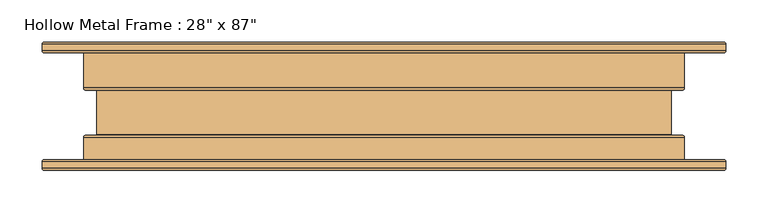
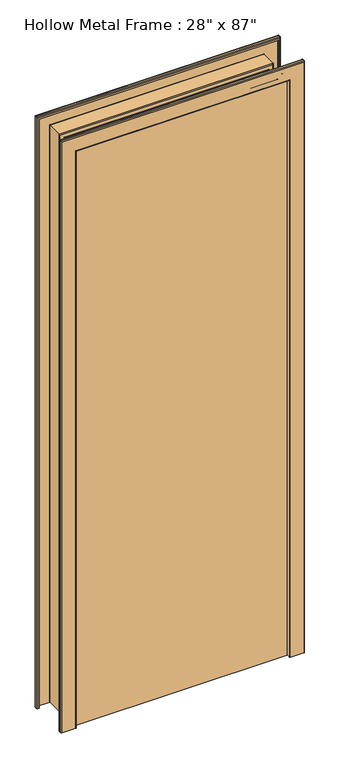
"""IFC4 building model written with IfcOpenShell, lengths in millimetres: door geometry."""

from ifc_helpers import new_model, si_unit, frame, origin, origin_with_axes, place, context, project, spatial, polyline, circle_curve, ellipse_curve, outline, extrude, source, transform, mapped, element, save
from ifc_brep_helpers import plane_surface, cylinder_surface, revolved_surface, advanced_brep


def door_ccd68c71(model_context):
    return source(origin(), model_context, "Body", "SolidModel", [
        advanced_brep(
        [(-403.82825, 63.5635, 0.0), (-406.4, 66.13525, 0.0), (-406.4, 73.66, 0.0), (-403.82825, 76.23175, 0.0), (-358.17175, 76.23175, 0.0), (-355.6, 73.66, 0.0), (-355.6, 21.68525, 0.0), (-354.584, 20.66925, 0.0), (-342.29675, 20.66925, 0.0), (-339.725, 18.0975, 0.0), (-339.725, -33.6931, 0.0), (-342.29675, -36.26485, 0.0), (-354.584, -36.26485, 0.0), (-355.6, -37.28085, 0.0), (-355.6, -73.5965, 0.0), (-358.17175, -76.16825, 0.0), (-403.82825, -76.16825, 0.0), (-406.4, -73.5965, 0.0), (-406.4, -66.07175, 0.0), (-403.82825, -63.5, 0.0), (-398.4625, -63.5, 0.0), (-398.4625, -65.05575, 0.0), (-403.82825, -65.05575, 0.0), (-404.84425, -66.07175, 0.0), (-404.84425, -73.5965, 0.0), (-403.82825, -74.6125, 0.0), (-358.17175, -74.6125, 0.0), (-357.15575, -73.5965, 0.0), (-357.15575, -37.28085, 0.0), (-354.584, -34.7091, 0.0), (-342.29675, -34.7091, 0.0), (-341.28075, -33.6931, 0.0), (-341.28075, 18.0975, 0.0), (-342.29675, 19.1135, 0.0), (-354.584, 19.1135, 0.0), (-357.15575, 21.68525, 0.0), (-357.15575, 73.66, 0.0), (-358.17175, 74.676, 0.0), (-403.82825, 74.676, 0.0), (-404.84425, 73.66, 0.0), (-404.84425, 66.13525, 0.0), (-403.82825, 65.11925, 0.0), (-398.4625, 65.11925, 0.0), (-398.4625, 63.5635, 0.0), (-403.82825, 63.5635, 2080.2282501), (-406.4, 66.13525, 2082.8000001), (-406.4, 73.66, 2082.8000001), (-403.82825, 76.23175, 2080.2282501), (403.82825, 76.23175, 2080.2282501), (403.82825, 76.23175, 0.0), (358.17175, 76.23175, 0.0), (358.17175, 76.23175, 2034.5717501), (-358.17175, 76.23175, 2034.5717501), (-355.6, 73.66, 2032.0000001), (-355.6, 21.68525, 2032.0000001), (-354.584, 20.66925, 2030.9840001), (354.584, 20.66925, 2030.9840001), (354.584, 20.66925, 0.0), (342.29675, 20.66925, 0.0), (342.29675, 20.66925, 2018.6967501), (-342.29675, 20.66925, 2018.6967501), (-339.725, 18.0975, 2016.1250001), (-339.725, -33.6931, 2016.1250001), (-342.29675, -36.26485, 2018.6967501), (342.29675, -36.26485, 2018.6967501), (342.29675, -36.26485, 0.0), (354.584, -36.26485, 0.0), (354.584, -36.26485, 2030.9840001), (-354.584, -36.26485, 2030.9840001), (-355.6, -37.28085, 2032.0000001), (-355.6, -73.5965, 2032.0000001), (-358.17175, -76.16825, 2034.5717501), (358.17175, -76.16825, 2034.5717501), (358.17175, -76.16825, 0.0), (403.82825, -76.16825, 0.0), (403.82825, -76.16825, 2080.2282501), (-403.82825, -76.16825, 2080.2282501), (-406.4, -73.5965, 2082.8000001), (-406.4, -66.07175, 2082.8000001), (-403.82825, -63.5, 2080.2282501), (403.82825, -63.5, 2080.2282501), (403.82825, -63.5, 0.0), (398.4625, -63.5, 0.0), (398.4625, -63.5, 2074.8625001), (-398.4625, -63.5, 2074.8625001), (-398.4625, -65.05575, 2074.8625001), (398.4625, -65.05575, 2074.8625001), (398.4625, -65.05575, 0.0), (403.82825, -65.05575, 0.0), (403.82825, -65.05575, 2080.2282501), (-403.82825, -65.05575, 2080.2282501), (-404.84425, -66.07175, 2081.2442501), (-404.84425, -73.5965, 2081.2442501), (-403.82825, -74.6125, 2080.2282501), (403.82825, -74.6125, 2080.2282501), (403.82825, -74.6125, 0.0), (358.17175, -74.6125, 0.0), (358.17175, -74.6125, 2034.5717501), (-358.17175, -74.6125, 2034.5717501), (-357.15575, -73.5965, 2033.5557501), (-357.15575, -37.28085, 2033.5557501), (-354.584, -34.7091, 2030.9840001), (354.584, -34.7091, 2030.9840001), (354.584, -34.7091, 0.0), (342.29675, -34.7091, 0.0), (342.29675, -34.7091, 2018.6967501), (-342.29675, -34.7091, 2018.6967501), (-341.28075, -33.6931, 2017.6807501), (-341.28075, 18.0975, 2017.6807501), (-342.29675, 19.1135, 2018.6967501), (342.29675, 19.1135, 2018.6967501), (342.29675, 19.1135, 0.0), (354.584, 19.1135, 0.0), (354.584, 19.1135, 2030.9840001), (-354.584, 19.1135, 2030.9840001), (-357.15575, 21.68525, 2033.5557501), (-357.15575, 73.66, 2033.5557501), (-358.17175, 74.676, 2034.5717501), (358.17175, 74.676, 2034.5717501), (358.17175, 74.676, 0.0), (403.82825, 74.676, 0.0), (403.82825, 74.676, 2080.2282501), (-403.82825, 74.676, 2080.2282501), (-404.84425, 73.66, 2081.2442501), (-404.84425, 66.13525, 2081.2442501), (-403.82825, 65.11925, 2080.2282501), (403.82825, 65.11925, 2080.2282501), (403.82825, 65.11925, 0.0), (398.4625, 65.11925, 0.0), (398.4625, 65.11925, 2074.8625001), (-398.4625, 65.11925, 2074.8625001), (-398.4625, 63.5635, 2074.8625001), (398.4625, 63.5635, 2074.8625001), (398.4625, 63.5635, 0.0), (403.82825, 63.5635, 0.0), (403.82825, 63.5635, 2080.2282501), (406.4, 66.13525, 2082.8000001), (406.4, 73.66, 2082.8000001), (355.6, 73.66, 2032.0000001), (355.6, 21.68525, 2032.0000001), (339.725, 18.0975, 2016.1250001), (339.725, -33.6931, 2016.1250001), (355.6, -37.28085, 2032.0000001), (355.6, -73.5965, 2032.0000001), (406.4, -73.5965, 2082.8000001), (406.4, -66.07175, 2082.8000001), (404.84425, -66.07175, 2081.2442501), (404.84425, -73.5965, 2081.2442501), (357.15575, -73.5965, 2033.5557501), (357.15575, -37.28085, 2033.5557501), (341.28075, -33.6931, 2017.6807501), (341.28075, 18.0975, 2017.6807501), (357.15575, 21.68525, 2033.5557501), (357.15575, 73.66, 2033.5557501), (404.84425, 73.66, 2081.2442501), (404.84425, 66.13525, 2081.2442501), (404.84425, 66.13525, 0.0), (404.84425, 73.66, 0.0), (357.15575, 73.66, 0.0), (357.15575, 21.68525, 0.0), (341.28075, 18.0975, 0.0), (341.28075, -33.6931, 0.0), (357.15575, -37.28085, 0.0), (357.15575, -73.5965, 0.0), (404.84425, -73.5965, 0.0), (404.84425, -66.07175, 0.0), (406.4, -66.07175, 0.0), (406.4, -73.5965, 0.0), (355.6, -73.5965, 0.0), (355.6, -37.28085, 0.0), (339.725, -33.6931, 0.0), (339.725, 18.0975, 0.0), (355.6, 21.68525, 0.0), (355.6, 73.66, 0.0), (406.4, 73.66, 0.0), (406.4, 66.13525, 0.0)],
        [
            (0, 1, circle_curve(frame((-403.82825, 66.13525, 0.0), z_axis=(0.0, 0.0, -1.0), x_axis=(0.0, -1.0, 0.0)), 2.57175)),
            (1, 2),
            (2, 3, circle_curve(frame((-403.82825, 73.66, 0.0), z_axis=(0.0, 0.0, -1.0), x_axis=(0.0, -1.0, 0.0)), 2.57175)),
            (3, 4),
            (4, 5, circle_curve(frame((-358.17175, 73.66, 0.0), z_axis=(0.0, 0.0, -1.0), x_axis=(0.0, -1.0, 0.0)), 2.57175)),
            (5, 6),
            (6, 7, circle_curve(frame((-354.584, 21.68525, 0.0), z_axis=(0.0, 0.0, 1.0), x_axis=(0.0, -1.0, 0.0)), 1.016)),
            (7, 8),
            (8, 9, circle_curve(frame((-342.29675, 18.0975, 0.0), z_axis=(0.0, 0.0, -1.0), x_axis=(0.0, -1.0, 0.0)), 2.57175)),
            (9, 10),
            (10, 11, circle_curve(frame((-342.29675, -33.6931, 0.0), z_axis=(0.0, 0.0, -1.0), x_axis=(0.0, -1.0, 0.0)), 2.57175)),
            (11, 12),
            (12, 13, circle_curve(frame((-354.584, -37.28085, 0.0), z_axis=(0.0, 0.0, 1.0), x_axis=(0.0, -1.0, 0.0)), 1.016)),
            (13, 14),
            (14, 15, circle_curve(frame((-358.17175, -73.5965, 0.0), z_axis=(0.0, 0.0, -1.0), x_axis=(0.0, -1.0, 0.0)), 2.57175)),
            (15, 16),
            (16, 17, circle_curve(frame((-403.82825, -73.5965, 0.0), z_axis=(0.0, 0.0, -1.0), x_axis=(0.0, -1.0, 0.0)), 2.57175)),
            (17, 18),
            (18, 19, circle_curve(frame((-403.82825, -66.07175, 0.0), z_axis=(0.0, 0.0, -1.0), x_axis=(0.0, -1.0, 0.0)), 2.57175)),
            (19, 20),
            (20, 21),
            (21, 22),
            (22, 23, circle_curve(frame((-403.82825, -66.07175, 0.0), z_axis=(0.0, 0.0, 1.0), x_axis=(0.0, -1.0, 0.0)), 1.016)),
            (23, 24),
            (24, 25, circle_curve(frame((-403.82825, -73.5965, 0.0), z_axis=(0.0, 0.0, 1.0), x_axis=(0.0, -1.0, 0.0)), 1.016)),
            (25, 26),
            (26, 27, circle_curve(frame((-358.17175, -73.5965, 0.0), z_axis=(0.0, 0.0, 1.0), x_axis=(0.0, -1.0, 0.0)), 1.016)),
            (27, 28),
            (28, 29, circle_curve(frame((-354.584, -37.28085, 0.0), z_axis=(0.0, 0.0, -1.0), x_axis=(0.0, -1.0, 0.0)), 2.57175)),
            (29, 30),
            (30, 31, circle_curve(frame((-342.29675, -33.6931, 0.0), z_axis=(0.0, 0.0, 1.0), x_axis=(0.0, -1.0, 0.0)), 1.016)),
            (31, 32),
            (32, 33, circle_curve(frame((-342.29675, 18.0975, 0.0), z_axis=(0.0, 0.0, 1.0), x_axis=(0.0, -1.0, 0.0)), 1.016)),
            (33, 34),
            (34, 35, circle_curve(frame((-354.584, 21.68525, 0.0), z_axis=(0.0, 0.0, -1.0), x_axis=(0.0, -1.0, 0.0)), 2.57175)),
            (35, 36),
            (36, 37, circle_curve(frame((-358.17175, 73.66, 0.0), z_axis=(0.0, 0.0, 1.0), x_axis=(0.0, -1.0, 0.0)), 1.016)),
            (37, 38),
            (38, 39, circle_curve(frame((-403.82825, 73.66, 0.0), z_axis=(0.0, 0.0, 1.0), x_axis=(0.0, -1.0, 0.0)), 1.016)),
            (39, 40),
            (40, 41, circle_curve(frame((-403.82825, 66.13525, 0.0), z_axis=(0.0, 0.0, 1.0), x_axis=(0.0, -1.0, 0.0)), 1.016)),
            (41, 42),
            (42, 43),
            (43, 0),
            (0, 44),
            (44, 45, ellipse_curve(frame((-403.82825, 66.13525, 2080.2282501), z_axis=(-0.7071067811865475, 0.0, -0.7071067811865475), x_axis=(0.7071067811865474, 0.0, -0.7071067811865476)), 3.6370037, 2.57175)),
            (45, 1),
            (45, 46),
            (46, 2),
            (46, 47, ellipse_curve(frame((-403.82825, 73.66, 2080.2282501), z_axis=(-0.7071067811865475, 0.0, -0.7071067811865475), x_axis=(0.7071067811865474, 0.0, -0.7071067811865476)), 3.6370037, 2.57175)),
            (47, 3),
            (47, 48),
            (48, 49),
            (49, 50),
            (50, 51),
            (51, 52),
            (52, 4),
            (52, 53, ellipse_curve(frame((-358.17175, 73.66, 2034.5717501), z_axis=(-0.7071067811865475, 0.0, -0.7071067811865475), x_axis=(0.7071067811865474, 0.0, -0.7071067811865476)), 3.6370037, 2.57175)),
            (53, 5),
            (53, 54),
            (54, 6),
            (54, 55, ellipse_curve(frame((-354.584, 21.68525, 2030.9840001), z_axis=(0.7071067811865475, 0.0, 0.7071067811865475), x_axis=(-0.7071067811865474, 0.0, 0.7071067811865476)), 1.436841, 1.016)),
            (55, 7),
            (55, 56),
            (56, 57),
            (57, 58),
            (58, 59),
            (59, 60),
            (60, 8),
            (60, 61, ellipse_curve(frame((-342.29675, 18.0975, 2018.6967501), z_axis=(-0.7071067811865475, 0.0, -0.7071067811865475), x_axis=(0.7071067811865474, 0.0, -0.7071067811865476)), 3.6370037, 2.57175)),
            (61, 9),
            (61, 62),
            (62, 10),
            (62, 63, ellipse_curve(frame((-342.29675, -33.6931, 2018.6967501), z_axis=(-0.7071067811865475, 0.0, -0.7071067811865475), x_axis=(0.7071067811865474, 0.0, -0.7071067811865476)), 3.6370037, 2.57175)),
            (63, 11),
            (63, 64),
            (64, 65),
            (65, 66),
            (66, 67),
            (67, 68),
            (68, 12),
            (68, 69, ellipse_curve(frame((-354.584, -37.28085, 2030.9840001), z_axis=(0.7071067811865475, 0.0, 0.7071067811865475), x_axis=(-0.7071067811865474, 0.0, 0.7071067811865476)), 1.436841, 1.016)),
            (69, 13),
            (69, 70),
            (70, 14),
            (70, 71, ellipse_curve(frame((-358.17175, -73.5965, 2034.5717501), z_axis=(-0.7071067811865475, 0.0, -0.7071067811865475), x_axis=(0.7071067811865474, 0.0, -0.7071067811865476)), 3.6370037, 2.57175)),
            (71, 15),
            (71, 72),
            (72, 73),
            (73, 74),
            (74, 75),
            (75, 76),
            (76, 16),
            (76, 77, ellipse_curve(frame((-403.82825, -73.5965, 2080.2282501), z_axis=(-0.7071067811865475, 0.0, -0.7071067811865475), x_axis=(0.7071067811865474, 0.0, -0.7071067811865476)), 3.6370037, 2.57175)),
            (77, 17),
            (77, 78),
            (78, 18),
            (78, 79, ellipse_curve(frame((-403.82825, -66.07175, 2080.2282501), z_axis=(-0.7071067811865475, 0.0, -0.7071067811865475), x_axis=(0.7071067811865474, 0.0, -0.7071067811865476)), 3.6370037, 2.57175)),
            (79, 19),
            (79, 80),
            (80, 81),
            (81, 82),
            (82, 83),
            (83, 84),
            (84, 20),
            (84, 85),
            (85, 21),
            (85, 86),
            (86, 87),
            (87, 88),
            (88, 89),
            (89, 90),
            (90, 22),
            (90, 91, ellipse_curve(frame((-403.82825, -66.07175, 2080.2282501), z_axis=(0.7071067811865475, 0.0, 0.7071067811865475), x_axis=(-0.7071067811865474, 0.0, 0.7071067811865476)), 1.436841, 1.016)),
            (91, 23),
            (91, 92),
            (92, 24),
            (92, 93, ellipse_curve(frame((-403.82825, -73.5965, 2080.2282501), z_axis=(0.7071067811865475, 0.0, 0.7071067811865475), x_axis=(-0.7071067811865474, 0.0, 0.7071067811865476)), 1.436841, 1.016)),
            (93, 25),
            (93, 94),
            (94, 95),
            (95, 96),
            (96, 97),
            (97, 98),
            (98, 26),
            (98, 99, ellipse_curve(frame((-358.17175, -73.5965, 2034.5717501), z_axis=(0.7071067811865475, 0.0, 0.7071067811865475), x_axis=(-0.7071067811865474, 0.0, 0.7071067811865476)), 1.436841, 1.016)),
            (99, 27),
            (99, 100),
            (100, 28),
            (100, 101, ellipse_curve(frame((-354.584, -37.28085, 2030.9840001), z_axis=(-0.7071067811865475, 0.0, -0.7071067811865475), x_axis=(0.7071067811865474, 0.0, -0.7071067811865476)), 3.6370037, 2.57175)),
            (101, 29),
            (101, 102),
            (102, 103),
            (103, 104),
            (104, 105),
            (105, 106),
            (106, 30),
            (106, 107, ellipse_curve(frame((-342.29675, -33.6931, 2018.6967501), z_axis=(0.7071067811865475, 0.0, 0.7071067811865475), x_axis=(-0.7071067811865474, 0.0, 0.7071067811865476)), 1.436841, 1.016)),
            (107, 31),
            (107, 108),
            (108, 32),
            (108, 109, ellipse_curve(frame((-342.29675, 18.0975, 2018.6967501), z_axis=(0.7071067811865475, 0.0, 0.7071067811865475), x_axis=(-0.7071067811865474, 0.0, 0.7071067811865476)), 1.436841, 1.016)),
            (109, 33),
            (109, 110),
            (110, 111),
            (111, 112),
            (112, 113),
            (113, 114),
            (114, 34),
            (114, 115, ellipse_curve(frame((-354.584, 21.68525, 2030.9840001), z_axis=(-0.7071067811865475, 0.0, -0.7071067811865475), x_axis=(0.7071067811865474, 0.0, -0.7071067811865476)), 3.6370037, 2.57175)),
            (115, 35),
            (115, 116),
            (116, 36),
            (116, 117, ellipse_curve(frame((-358.17175, 73.66, 2034.5717501), z_axis=(0.7071067811865475, 0.0, 0.7071067811865475), x_axis=(-0.7071067811865474, 0.0, 0.7071067811865476)), 1.436841, 1.016)),
            (117, 37),
            (117, 118),
            (118, 119),
            (119, 120),
            (120, 121),
            (121, 122),
            (122, 38),
            (122, 123, ellipse_curve(frame((-403.82825, 73.66, 2080.2282501), z_axis=(0.7071067811865475, 0.0, 0.7071067811865475), x_axis=(-0.7071067811865474, 0.0, 0.7071067811865476)), 1.436841, 1.016)),
            (123, 39),
            (123, 124),
            (124, 40),
            (124, 125, ellipse_curve(frame((-403.82825, 66.13525, 2080.2282501), z_axis=(0.7071067811865475, 0.0, 0.7071067811865475), x_axis=(-0.7071067811865474, 0.0, 0.7071067811865476)), 1.436841, 1.016)),
            (125, 41),
            (125, 126),
            (126, 127),
            (127, 128),
            (128, 129),
            (129, 130),
            (130, 42),
            (130, 131),
            (131, 43),
            (131, 132),
            (132, 133),
            (133, 134),
            (134, 135),
            (135, 44),
            (135, 136, ellipse_curve(frame((403.82825, 66.13525, 2080.2282501), z_axis=(-0.7071067811865475, 0.0, 0.7071067811865475), x_axis=(-0.7071067811865476, 0.0, -0.7071067811865474)), 3.6370037, 2.57175)),
            (136, 45),
            (136, 137),
            (137, 46),
            (137, 48, ellipse_curve(frame((403.82825, 73.66, 2080.2282501), z_axis=(-0.7071067811865475, 0.0, 0.7071067811865475), x_axis=(-0.7071067811865476, 0.0, -0.7071067811865474)), 3.6370037, 2.57175)),
            (51, 138, ellipse_curve(frame((358.17175, 73.66, 2034.5717501), z_axis=(-0.7071067811865475, 0.0, 0.7071067811865475), x_axis=(-0.7071067811865476, 0.0, -0.7071067811865474)), 3.6370037, 2.57175)),
            (138, 53),
            (138, 139),
            (139, 54),
            (139, 56, ellipse_curve(frame((354.584, 21.68525, 2030.9840001), z_axis=(0.7071067811865475, 0.0, -0.7071067811865475), x_axis=(0.7071067811865476, 0.0, 0.7071067811865474)), 1.436841, 1.016)),
            (59, 140, ellipse_curve(frame((342.29675, 18.0975, 2018.6967501), z_axis=(-0.7071067811865475, 0.0, 0.7071067811865475), x_axis=(-0.7071067811865476, 0.0, -0.7071067811865474)), 3.6370037, 2.57175)),
            (140, 61),
            (140, 141),
            (141, 62),
            (141, 64, ellipse_curve(frame((342.29675, -33.6931, 2018.6967501), z_axis=(-0.7071067811865475, 0.0, 0.7071067811865475), x_axis=(-0.7071067811865476, 0.0, -0.7071067811865474)), 3.6370037, 2.57175)),
            (67, 142, ellipse_curve(frame((354.584, -37.28085, 2030.9840001), z_axis=(0.7071067811865475, 0.0, -0.7071067811865475), x_axis=(0.7071067811865476, 0.0, 0.7071067811865474)), 1.436841, 1.016)),
            (142, 69),
            (142, 143),
            (143, 70),
            (143, 72, ellipse_curve(frame((358.17175, -73.5965, 2034.5717501), z_axis=(-0.7071067811865475, 0.0, 0.7071067811865475), x_axis=(-0.7071067811865476, 0.0, -0.7071067811865474)), 3.6370037, 2.57175)),
            (75, 144, ellipse_curve(frame((403.82825, -73.5965, 2080.2282501), z_axis=(-0.7071067811865475, 0.0, 0.7071067811865475), x_axis=(-0.7071067811865476, 0.0, -0.7071067811865474)), 3.6370037, 2.57175)),
            (144, 77),
            (144, 145),
            (145, 78),
            (145, 80, ellipse_curve(frame((403.82825, -66.07175, 2080.2282501), z_axis=(-0.7071067811865475, 0.0, 0.7071067811865475), x_axis=(-0.7071067811865476, 0.0, -0.7071067811865474)), 3.6370037, 2.57175)),
            (83, 86),
            (89, 146, ellipse_curve(frame((403.82825, -66.07175, 2080.2282501), z_axis=(0.7071067811865475, 0.0, -0.7071067811865475), x_axis=(0.7071067811865476, 0.0, 0.7071067811865474)), 1.436841, 1.016)),
            (146, 91),
            (146, 147),
            (147, 92),
            (147, 94, ellipse_curve(frame((403.82825, -73.5965, 2080.2282501), z_axis=(0.7071067811865475, 0.0, -0.7071067811865475), x_axis=(0.7071067811865476, 0.0, 0.7071067811865474)), 1.436841, 1.016)),
            (97, 148, ellipse_curve(frame((358.17175, -73.5965, 2034.5717501), z_axis=(0.7071067811865475, 0.0, -0.7071067811865475), x_axis=(0.7071067811865476, 0.0, 0.7071067811865474)), 1.436841, 1.016)),
            (148, 99),
            (148, 149),
            (149, 100),
            (149, 102, ellipse_curve(frame((354.584, -37.28085, 2030.9840001), z_axis=(-0.7071067811865475, 0.0, 0.7071067811865475), x_axis=(-0.7071067811865476, 0.0, -0.7071067811865474)), 3.6370037, 2.57175)),
            (105, 150, ellipse_curve(frame((342.29675, -33.6931, 2018.6967501), z_axis=(0.7071067811865475, 0.0, -0.7071067811865475), x_axis=(0.7071067811865476, 0.0, 0.7071067811865474)), 1.436841, 1.016)),
            (150, 107),
            (150, 151),
            (151, 108),
            (151, 110, ellipse_curve(frame((342.29675, 18.0975, 2018.6967501), z_axis=(0.7071067811865475, 0.0, -0.7071067811865475), x_axis=(0.7071067811865476, 0.0, 0.7071067811865474)), 1.436841, 1.016)),
            (113, 152, ellipse_curve(frame((354.584, 21.68525, 2030.9840001), z_axis=(-0.7071067811865475, 0.0, 0.7071067811865475), x_axis=(-0.7071067811865476, 0.0, -0.7071067811865474)), 3.6370037, 2.57175)),
            (152, 115),
            (152, 153),
            (153, 116),
            (153, 118, ellipse_curve(frame((358.17175, 73.66, 2034.5717501), z_axis=(0.7071067811865475, 0.0, -0.7071067811865475), x_axis=(0.7071067811865476, 0.0, 0.7071067811865474)), 1.436841, 1.016)),
            (121, 154, ellipse_curve(frame((403.82825, 73.66, 2080.2282501), z_axis=(0.7071067811865475, 0.0, -0.7071067811865475), x_axis=(0.7071067811865476, 0.0, 0.7071067811865474)), 1.436841, 1.016)),
            (154, 123),
            (154, 155),
            (155, 124),
            (155, 126, ellipse_curve(frame((403.82825, 66.13525, 2080.2282501), z_axis=(0.7071067811865475, 0.0, -0.7071067811865475), x_axis=(0.7071067811865476, 0.0, 0.7071067811865474)), 1.436841, 1.016)),
            (129, 132),
            (133, 128),
            (127, 156, circle_curve(frame((403.82825, 66.13525, 0.0), z_axis=(0.0, 0.0, 1.0), x_axis=(0.0, -1.0, 0.0)), 1.016)),
            (156, 157),
            (157, 120, circle_curve(frame((403.82825, 73.66, 0.0), z_axis=(0.0, 0.0, 1.0), x_axis=(0.0, -1.0, 0.0)), 1.016)),
            (119, 158, circle_curve(frame((358.17175, 73.66, 0.0), z_axis=(0.0, 0.0, 1.0), x_axis=(0.0, -1.0, 0.0)), 1.016)),
            (158, 159),
            (159, 112, circle_curve(frame((354.584, 21.68525, 0.0), z_axis=(0.0, 0.0, -1.0), x_axis=(0.0, -1.0, 0.0)), 2.57175)),
            (111, 160, circle_curve(frame((342.29675, 18.0975, 0.0), z_axis=(0.0, 0.0, 1.0), x_axis=(0.0, -1.0, 0.0)), 1.016)),
            (160, 161),
            (161, 104, circle_curve(frame((342.29675, -33.6931, 0.0), z_axis=(0.0, 0.0, 1.0), x_axis=(0.0, -1.0, 0.0)), 1.016)),
            (103, 162, circle_curve(frame((354.584, -37.28085, 0.0), z_axis=(0.0, 0.0, -1.0), x_axis=(0.0, -1.0, 0.0)), 2.57175)),
            (162, 163),
            (163, 96, circle_curve(frame((358.17175, -73.5965, 0.0), z_axis=(0.0, 0.0, 1.0), x_axis=(0.0, -1.0, 0.0)), 1.016)),
            (95, 164, circle_curve(frame((403.82825, -73.5965, 0.0), z_axis=(0.0, 0.0, 1.0), x_axis=(0.0, -1.0, 0.0)), 1.016)),
            (164, 165),
            (165, 88, circle_curve(frame((403.82825, -66.07175, 0.0), z_axis=(0.0, 0.0, 1.0), x_axis=(0.0, -1.0, 0.0)), 1.016)),
            (87, 82),
            (81, 166, circle_curve(frame((403.82825, -66.07175, 0.0), z_axis=(0.0, 0.0, -1.0), x_axis=(0.0, -1.0, 0.0)), 2.57175)),
            (166, 167),
            (167, 74, circle_curve(frame((403.82825, -73.5965, 0.0), z_axis=(0.0, 0.0, -1.0), x_axis=(0.0, -1.0, 0.0)), 2.57175)),
            (73, 168, circle_curve(frame((358.17175, -73.5965, 0.0), z_axis=(0.0, 0.0, -1.0), x_axis=(0.0, -1.0, 0.0)), 2.57175)),
            (168, 169),
            (169, 66, circle_curve(frame((354.584, -37.28085, 0.0), z_axis=(0.0, 0.0, 1.0), x_axis=(0.0, -1.0, 0.0)), 1.016)),
            (65, 170, circle_curve(frame((342.29675, -33.6931, 0.0), z_axis=(0.0, 0.0, -1.0), x_axis=(0.0, -1.0, 0.0)), 2.57175)),
            (170, 171),
            (171, 58, circle_curve(frame((342.29675, 18.0975, 0.0), z_axis=(0.0, 0.0, -1.0), x_axis=(0.0, -1.0, 0.0)), 2.57175)),
            (57, 172, circle_curve(frame((354.584, 21.68525, 0.0), z_axis=(0.0, 0.0, 1.0), x_axis=(0.0, -1.0, 0.0)), 1.016)),
            (172, 173),
            (173, 50, circle_curve(frame((358.17175, 73.66, 0.0), z_axis=(0.0, 0.0, -1.0), x_axis=(0.0, -1.0, 0.0)), 2.57175)),
            (49, 174, circle_curve(frame((403.82825, 73.66, 0.0), z_axis=(0.0, 0.0, -1.0), x_axis=(0.0, -1.0, 0.0)), 2.57175)),
            (174, 175),
            (175, 134, circle_curve(frame((403.82825, 66.13525, 0.0), z_axis=(0.0, 0.0, -1.0), x_axis=(0.0, -1.0, 0.0)), 2.57175)),
            (175, 136),
            (174, 137),
            (173, 138),
            (172, 139),
            (171, 140),
            (170, 141),
            (169, 142),
            (168, 143),
            (167, 144),
            (166, 145),
            (165, 146),
            (164, 147),
            (163, 148),
            (162, 149),
            (161, 150),
            (160, 151),
            (159, 152),
            (158, 153),
            (157, 154),
            (156, 155),
        ],
        [
            plane_surface(frame((-366.7125, -63.5, 0.0), z_axis=(0.0, 0.0, -1.0), x_axis=(1.0, 0.0, 0.0))),
            cylinder_surface(frame((-403.82825, 66.13525, 0.0), z_axis=(0.0, 0.0, -1.0), x_axis=(0.0, -1.0, 0.0)), 2.57175),
            plane_surface(frame((-406.4, 66.13525, 0.0), z_axis=(-1.0, 0.0, 0.0), x_axis=(0.0, 0.0, 1.0))),
            cylinder_surface(frame((-403.82825, 73.66, 0.0), z_axis=(0.0, 0.0, -1.0), x_axis=(0.0, -1.0, 0.0)), 2.57175),
            plane_surface(frame((-403.82825, 76.23175, 0.0), z_axis=(0.0, 1.0, 0.0), x_axis=(0.0, 0.0, 1.0))),
            cylinder_surface(frame((-358.17175, 73.66, 0.0), z_axis=(0.0, 0.0, -1.0), x_axis=(0.0, -1.0, 0.0)), 2.57175),
            plane_surface(frame((-355.6, 73.66, 0.0), z_axis=(1.0, 0.0, 0.0), x_axis=(0.0, 0.0, 1.0))),
            revolved_surface(polyline([(-354.584, 20.669249999999998, 2032.0000001145868), (-354.584, 20.669249999999998, 0.0)]), (-354.584, 21.68525, 0.0), (0.0, 0.0, 1.0)),
            plane_surface(frame((-354.584, 20.66925, 0.0), z_axis=(0.0, 1.0, 0.0), x_axis=(0.0, 0.0, 1.0))),
            cylinder_surface(frame((-342.29675, 18.0975, 0.0), z_axis=(0.0, 0.0, -1.0), x_axis=(0.0, -1.0, 0.0)), 2.57175),
            plane_surface(frame((-339.725, 18.0975, 0.0), z_axis=(1.0, 0.0, 0.0), x_axis=(0.0, 0.0, 1.0))),
            cylinder_surface(frame((-342.29675, -33.6931, 0.0), z_axis=(0.0, 0.0, -1.0), x_axis=(0.0, -1.0, 0.0)), 2.57175),
            plane_surface(frame((-342.29675, -36.26485, 0.0), z_axis=(0.0, -1.0, 0.0), x_axis=(0.0, 0.0, 1.0))),
            revolved_surface(polyline([(-354.584, -38.29685, 2032.0000001145868), (-354.584, -38.29685, 0.0)]), (-354.584, -37.28085, 0.0), (0.0, 0.0, 1.0)),
            plane_surface(frame((-355.6, -37.28085, 0.0), z_axis=(1.0, 0.0, 0.0), x_axis=(0.0, 0.0, 1.0))),
            cylinder_surface(frame((-358.17175, -73.5965, 0.0), z_axis=(0.0, 0.0, -1.0), x_axis=(0.0, -1.0, 0.0)), 2.57175),
            plane_surface(frame((-358.17175, -76.16825, 0.0), z_axis=(0.0, -1.0, 0.0), x_axis=(0.0, 0.0, 1.0))),
            cylinder_surface(frame((-403.82825, -73.5965, 0.0), z_axis=(0.0, 0.0, -1.0), x_axis=(0.0, -1.0, 0.0)), 2.57175),
            plane_surface(frame((-406.4, -73.5965, 0.0), z_axis=(-1.0, 0.0, 0.0), x_axis=(0.0, 0.0, 1.0))),
            cylinder_surface(frame((-403.82825, -66.07175, 0.0), z_axis=(0.0, 0.0, -1.0), x_axis=(0.0, -1.0, 0.0)), 2.57175),
            plane_surface(frame((-403.82825, -63.5, 0.0), z_axis=(0.0, 1.0, 0.0), x_axis=(0.0, 0.0, 1.0))),
            plane_surface(frame((-398.4625, -63.5, 0.0), z_axis=(1.0, 0.0, 0.0), x_axis=(0.0, 0.0, 1.0))),
            plane_surface(frame((-398.4625, -65.05575, 0.0), z_axis=(0.0, -1.0, 0.0), x_axis=(0.0, 0.0, 1.0))),
            revolved_surface(polyline([(-403.82825, -67.08775, 2081.244250114587), (-403.82825, -67.08775, 0.0)]), (-403.82825, -66.07175, 0.0), (0.0, 0.0, 1.0)),
            plane_surface(frame((-404.84425, -66.07175, 0.0), z_axis=(1.0, 0.0, 0.0), x_axis=(0.0, 0.0, 1.0))),
            revolved_surface(polyline([(-403.82825, -74.61250000000001, 2081.244250114587), (-403.82825, -74.61250000000001, 0.0)]), (-403.82825, -73.5965, 0.0), (0.0, 0.0, 1.0)),
            plane_surface(frame((-403.82825, -74.6125, 0.0), z_axis=(0.0, 1.0, 0.0), x_axis=(0.0, 0.0, 1.0))),
            revolved_surface(polyline([(-358.17175, -74.61250000000001, 2035.5877501145867), (-358.17175, -74.61250000000001, 0.0)]), (-358.17175, -73.5965, 0.0), (0.0, 0.0, 1.0)),
            plane_surface(frame((-357.15575, -73.5965, 0.0), z_axis=(-1.0, 0.0, 0.0), x_axis=(0.0, 0.0, 1.0))),
            cylinder_surface(frame((-354.584, -37.28085, 0.0), z_axis=(0.0, 0.0, -1.0), x_axis=(0.0, -1.0, 0.0)), 2.57175),
            plane_surface(frame((-354.584, -34.7091, 0.0), z_axis=(0.0, 1.0, 0.0), x_axis=(0.0, 0.0, 1.0))),
            revolved_surface(polyline([(-342.29675, -34.7091, 2019.7127501145867), (-342.29675, -34.7091, 0.0)]), (-342.29675, -33.6931, 0.0), (0.0, 0.0, 1.0)),
            plane_surface(frame((-341.28075, -33.6931, 0.0), z_axis=(-1.0, 0.0, 0.0), x_axis=(0.0, 0.0, 1.0))),
            revolved_surface(polyline([(-342.29675, 17.0815, 2019.7127501145867), (-342.29675, 17.0815, 0.0)]), (-342.29675, 18.0975, 0.0), (0.0, 0.0, 1.0)),
            plane_surface(frame((-342.29675, 19.1135, 0.0), z_axis=(0.0, -1.0, 0.0), x_axis=(0.0, 0.0, 1.0))),
            cylinder_surface(frame((-354.584, 21.68525, 0.0), z_axis=(0.0, 0.0, -1.0), x_axis=(0.0, -1.0, 0.0)), 2.57175),
            plane_surface(frame((-357.15575, 21.68525, 0.0), z_axis=(-1.0, 0.0, 0.0), x_axis=(0.0, 0.0, 1.0))),
            revolved_surface(polyline([(-358.17175, 72.64399999999999, 2035.5877501145867), (-358.17175, 72.64399999999999, 0.0)]), (-358.17175, 73.66, 0.0), (0.0, 0.0, 1.0)),
            plane_surface(frame((-358.17175, 74.676, 0.0), z_axis=(0.0, -1.0, 0.0), x_axis=(0.0, 0.0, 1.0))),
            revolved_surface(polyline([(-403.82825, 72.64399999999999, 2081.244250114587), (-403.82825, 72.64399999999999, 0.0)]), (-403.82825, 73.66, 0.0), (0.0, 0.0, 1.0)),
            plane_surface(frame((-404.84425, 73.66, 0.0), z_axis=(1.0, 0.0, 0.0), x_axis=(0.0, 0.0, 1.0))),
            revolved_surface(polyline([(-403.82825, 65.11925, 2081.244250114587), (-403.82825, 65.11925, 0.0)]), (-403.82825, 66.13525, 0.0), (0.0, 0.0, 1.0)),
            plane_surface(frame((-403.82825, 65.11925, 0.0), z_axis=(0.0, 1.0, 0.0), x_axis=(0.0, 0.0, 1.0))),
            plane_surface(frame((-398.4625, 65.11925, 0.0), z_axis=(1.0, 0.0, 0.0), x_axis=(0.0, 0.0, 1.0))),
            plane_surface(frame((-398.4625, 63.5635, 0.0), z_axis=(0.0, -1.0, 0.0), x_axis=(0.0, 0.0, 1.0))),
            cylinder_surface(frame((-366.7125, 66.13525, 2080.2282501), z_axis=(-1.0, 0.0, 0.0), x_axis=(0.0, -1.0, 0.0)), 2.57175),
            plane_surface(frame((-406.4, 66.13525, 2082.8000001), z_axis=(0.0, 0.0, 1.0), x_axis=(1.0, 0.0, 0.0))),
            cylinder_surface(frame((-366.7125, 73.66, 2080.2282501), z_axis=(-1.0, 0.0, 0.0), x_axis=(0.0, -1.0, 0.0)), 2.57175),
            cylinder_surface(frame((-366.7125, 73.66, 2034.5717501), z_axis=(-1.0, 0.0, 0.0), x_axis=(0.0, -1.0, 0.0)), 2.57175),
            plane_surface(frame((-355.6, 73.66, 2032.0000001), z_axis=(0.0, 0.0, -1.0), x_axis=(1.0, 0.0, 0.0))),
            revolved_surface(polyline([(355.60000001458684, 20.669249999999998, 2030.9840001), (-355.60000001458684, 20.669249999999998, 2030.9840001)]), (-366.7125, 21.68525, 2030.9840001), (1.0, 0.0, 0.0)),
            cylinder_surface(frame((-366.7125, 18.0975, 2018.6967501), z_axis=(-1.0, 0.0, 0.0), x_axis=(0.0, -1.0, 0.0)), 2.57175),
            plane_surface(frame((-339.725, 18.0975, 2016.1250001), z_axis=(0.0, 0.0, -1.0), x_axis=(1.0, 0.0, 0.0))),
            cylinder_surface(frame((-366.7125, -33.6931, 2018.6967501), z_axis=(-1.0, 0.0, 0.0), x_axis=(0.0, -1.0, 0.0)), 2.57175),
            revolved_surface(polyline([(355.60000001458684, -38.29685, 2030.9840001), (-355.60000001458684, -38.29685, 2030.9840001)]), (-366.7125, -37.28085, 2030.9840001), (1.0, 0.0, 0.0)),
            plane_surface(frame((-355.6, -37.28085, 2032.0000001), z_axis=(0.0, 0.0, -1.0), x_axis=(1.0, 0.0, 0.0))),
            cylinder_surface(frame((-366.7125, -73.5965, 2034.5717501), z_axis=(-1.0, 0.0, 0.0), x_axis=(0.0, -1.0, 0.0)), 2.57175),
            cylinder_surface(frame((-366.7125, -73.5965, 2080.2282501), z_axis=(-1.0, 0.0, 0.0), x_axis=(0.0, -1.0, 0.0)), 2.57175),
            plane_surface(frame((-406.4, -73.5965, 2082.8000001), z_axis=(0.0, 0.0, 1.0), x_axis=(1.0, 0.0, 0.0))),
            cylinder_surface(frame((-366.7125, -66.07175, 2080.2282501), z_axis=(-1.0, 0.0, 0.0), x_axis=(0.0, -1.0, 0.0)), 2.57175),
            plane_surface(frame((-398.4625, -63.5, 2074.8625001), z_axis=(0.0, 0.0, -1.0), x_axis=(1.0, 0.0, 0.0))),
            revolved_surface(polyline([(404.8442500145869, -67.08775, 2080.2282501), (-404.84425001458686, -67.08775, 2080.2282501)]), (-366.7125, -66.07175, 2080.2282501), (1.0, 0.0, 0.0)),
            plane_surface(frame((-404.84425, -66.07175, 2081.2442501), z_axis=(0.0, 0.0, -1.0), x_axis=(1.0, 0.0, 0.0))),
            revolved_surface(polyline([(404.8442500145869, -74.61250000000001, 2080.2282501), (-404.84425001458686, -74.61250000000001, 2080.2282501)]), (-366.7125, -73.5965, 2080.2282501), (1.0, 0.0, 0.0)),
            revolved_surface(polyline([(359.18775001458687, -74.61250000000001, 2034.5717501), (-359.1877500145868, -74.61250000000001, 2034.5717501)]), (-366.7125, -73.5965, 2034.5717501), (1.0, 0.0, 0.0)),
            plane_surface(frame((-357.15575, -73.5965, 2033.5557501), z_axis=(0.0, 0.0, 1.0), x_axis=(1.0, 0.0, 0.0))),
            cylinder_surface(frame((-366.7125, -37.28085, 2030.9840001), z_axis=(-1.0, 0.0, 0.0), x_axis=(0.0, -1.0, 0.0)), 2.57175),
            revolved_surface(polyline([(343.31275001458687, -34.7091, 2018.6967501), (-343.3127500145868, -34.7091, 2018.6967501)]), (-366.7125, -33.6931, 2018.6967501), (1.0, 0.0, 0.0)),
            plane_surface(frame((-341.28075, -33.6931, 2017.6807501), z_axis=(0.0, 0.0, 1.0), x_axis=(1.0, 0.0, 0.0))),
            revolved_surface(polyline([(343.31275001458687, 17.0815, 2018.6967501), (-343.3127500145868, 17.0815, 2018.6967501)]), (-366.7125, 18.0975, 2018.6967501), (1.0, 0.0, 0.0)),
            cylinder_surface(frame((-366.7125, 21.68525, 2030.9840001), z_axis=(-1.0, 0.0, 0.0), x_axis=(0.0, -1.0, 0.0)), 2.57175),
            plane_surface(frame((-357.15575, 21.68525, 2033.5557501), z_axis=(0.0, 0.0, 1.0), x_axis=(1.0, 0.0, 0.0))),
            revolved_surface(polyline([(359.18775001458687, 72.64399999999999, 2034.5717501), (-359.1877500145868, 72.64399999999999, 2034.5717501)]), (-366.7125, 73.66, 2034.5717501), (1.0, 0.0, 0.0)),
            revolved_surface(polyline([(404.8442500145869, 72.64399999999999, 2080.2282501), (-404.84425001458686, 72.64399999999999, 2080.2282501)]), (-366.7125, 73.66, 2080.2282501), (1.0, 0.0, 0.0)),
            plane_surface(frame((-404.84425, 73.66, 2081.2442501), z_axis=(0.0, 0.0, -1.0), x_axis=(1.0, 0.0, 0.0))),
            revolved_surface(polyline([(404.8442500145869, 65.11925, 2080.2282501), (-404.84425001458686, 65.11925, 2080.2282501)]), (-366.7125, 66.13525, 2080.2282501), (1.0, 0.0, 0.0)),
            plane_surface(frame((-398.4625, 65.11925, 2074.8625001), z_axis=(0.0, 0.0, -1.0), x_axis=(1.0, 0.0, 0.0))),
            plane_surface(frame((366.7125, -63.5, 0.0), z_axis=(0.0, 0.0, -1.0), x_axis=(-1.0, 0.0, 0.0))),
            cylinder_surface(frame((403.82825, 66.13525, 2043.1125001), z_axis=(0.0, 0.0, 1.0), x_axis=(0.0, -1.0, 0.0)), 2.57175),
            plane_surface(frame((406.4, 66.13525, 2082.8000001), z_axis=(1.0, 0.0, 0.0), x_axis=(0.0, 0.0, -1.0))),
            cylinder_surface(frame((403.82825, 73.66, 2043.1125001), z_axis=(0.0, 0.0, 1.0), x_axis=(0.0, -1.0, 0.0)), 2.57175),
            cylinder_surface(frame((358.17175, 73.66, 2043.1125001), z_axis=(0.0, 0.0, 1.0), x_axis=(0.0, -1.0, 0.0)), 2.57175),
            plane_surface(frame((355.6, 73.66, 2032.0000001), z_axis=(-1.0, 0.0, 0.0), x_axis=(0.0, 0.0, -1.0))),
            revolved_surface(polyline([(354.584, 20.669249999999998, 0.0), (354.584, 20.669249999999998, 2032.0000001145868)]), (354.584, 21.68525, 2043.1125001), (0.0, 0.0, -1.0)),
            cylinder_surface(frame((342.29675, 18.0975, 2043.1125001), z_axis=(0.0, 0.0, 1.0), x_axis=(0.0, -1.0, 0.0)), 2.57175),
            plane_surface(frame((339.725, 18.0975, 2016.1250001), z_axis=(-1.0, 0.0, 0.0), x_axis=(0.0, 0.0, -1.0))),
            cylinder_surface(frame((342.29675, -33.6931, 2043.1125001), z_axis=(0.0, 0.0, 1.0), x_axis=(0.0, -1.0, 0.0)), 2.57175),
            revolved_surface(polyline([(354.584, -38.29685, 0.0), (354.584, -38.29685, 2032.0000001145868)]), (354.584, -37.28085, 2043.1125001), (0.0, 0.0, -1.0)),
            plane_surface(frame((355.6, -37.28085, 2032.0000001), z_axis=(-1.0, 0.0, 0.0), x_axis=(0.0, 0.0, -1.0))),
            cylinder_surface(frame((358.17175, -73.5965, 2043.1125001), z_axis=(0.0, 0.0, 1.0), x_axis=(0.0, -1.0, 0.0)), 2.57175),
            cylinder_surface(frame((403.82825, -73.5965, 2043.1125001), z_axis=(0.0, 0.0, 1.0), x_axis=(0.0, -1.0, 0.0)), 2.57175),
            plane_surface(frame((406.4, -73.5965, 2082.8000001), z_axis=(1.0, 0.0, 0.0), x_axis=(0.0, 0.0, -1.0))),
            cylinder_surface(frame((403.82825, -66.07175, 2043.1125001), z_axis=(0.0, 0.0, 1.0), x_axis=(0.0, -1.0, 0.0)), 2.57175),
            plane_surface(frame((398.4625, -63.5, 2074.8625001), z_axis=(-1.0, 0.0, 0.0), x_axis=(0.0, 0.0, -1.0))),
            revolved_surface(polyline([(403.82825, -67.08775, 0.0), (403.82825, -67.08775, 2081.244250114587)]), (403.82825, -66.07175, 2043.1125001), (0.0, 0.0, -1.0)),
            plane_surface(frame((404.84425, -66.07175, 2081.2442501), z_axis=(-1.0, 0.0, 0.0), x_axis=(0.0, 0.0, -1.0))),
            revolved_surface(polyline([(403.82825, -74.61250000000001, 0.0), (403.82825, -74.61250000000001, 2081.244250114587)]), (403.82825, -73.5965, 2043.1125001), (0.0, 0.0, -1.0)),
            revolved_surface(polyline([(358.17175, -74.61250000000001, 0.0), (358.17175, -74.61250000000001, 2035.5877501145867)]), (358.17175, -73.5965, 2043.1125001), (0.0, 0.0, -1.0)),
            plane_surface(frame((357.15575, -73.5965, 2033.5557501), z_axis=(1.0, 0.0, 0.0), x_axis=(0.0, 0.0, -1.0))),
            cylinder_surface(frame((354.584, -37.28085, 2043.1125001), z_axis=(0.0, 0.0, 1.0), x_axis=(0.0, -1.0, 0.0)), 2.57175),
            revolved_surface(polyline([(342.29675, -34.7091, 0.0), (342.29675, -34.7091, 2019.7127501145867)]), (342.29675, -33.6931, 2043.1125001), (0.0, 0.0, -1.0)),
            plane_surface(frame((341.28075, -33.6931, 2017.6807501), z_axis=(1.0, 0.0, 0.0), x_axis=(0.0, 0.0, -1.0))),
            revolved_surface(polyline([(342.29675, 17.0815, 0.0), (342.29675, 17.0815, 2019.7127501145867)]), (342.29675, 18.0975, 2043.1125001), (0.0, 0.0, -1.0)),
            cylinder_surface(frame((354.584, 21.68525, 2043.1125001), z_axis=(0.0, 0.0, 1.0), x_axis=(0.0, -1.0, 0.0)), 2.57175),
            plane_surface(frame((357.15575, 21.68525, 2033.5557501), z_axis=(1.0, 0.0, 0.0), x_axis=(0.0, 0.0, -1.0))),
            revolved_surface(polyline([(358.17175, 72.64399999999999, 0.0), (358.17175, 72.64399999999999, 2035.5877501145867)]), (358.17175, 73.66, 2043.1125001), (0.0, 0.0, -1.0)),
            revolved_surface(polyline([(403.82825, 72.64399999999999, 0.0), (403.82825, 72.64399999999999, 2081.244250114587)]), (403.82825, 73.66, 2043.1125001), (0.0, 0.0, -1.0)),
            plane_surface(frame((404.84425, 73.66, 2081.2442501), z_axis=(-1.0, 0.0, 0.0), x_axis=(0.0, 0.0, -1.0))),
            revolved_surface(polyline([(403.82825, 65.11925, 0.0), (403.82825, 65.11925, 2081.244250114587)]), (403.82825, 66.13525, 2043.1125001), (0.0, 0.0, -1.0)),
            plane_surface(frame((398.4625, 65.11925, 2074.8625001), z_axis=(-1.0, 0.0, 0.0), x_axis=(0.0, 0.0, -1.0))),
        ],
        [
            (0, [[1, 2, 3, 4, 5, 6, 7, 8, 9, 10, 11, 12, 13, 14, 15, 16, 17, 18, 19, 20, 21, 22, 23, 24, 25, 26, 27, 28, 29, 30, 31, 32, 33, 34, 35, 36, 37, 38, 39, 40, 41, 42, 43, 44]]),
            (1, [[-1, 45, 46, 47]]),
            (2, [[-2, -47, 48, 49]]),
            (3, [[-3, -49, 50, 51]]),
            (4, [[-4, -51, 52, 53, 54, 55, 56, 57]]),
            (5, [[-5, -57, 58, 59]]),
            (6, [[-6, -59, 60, 61]]),
            (7, [[-7, -61, 62, 63]]),
            (8, [[-8, -63, 64, 65, 66, 67, 68, 69]]),
            (9, [[-9, -69, 70, 71]]),
            (10, [[-10, -71, 72, 73]]),
            (11, [[-11, -73, 74, 75]]),
            (12, [[-12, -75, 76, 77, 78, 79, 80, 81]]),
            (13, [[-13, -81, 82, 83]]),
            (14, [[-14, -83, 84, 85]]),
            (15, [[-15, -85, 86, 87]]),
            (16, [[-16, -87, 88, 89, 90, 91, 92, 93]]),
            (17, [[-17, -93, 94, 95]]),
            (18, [[-18, -95, 96, 97]]),
            (19, [[-19, -97, 98, 99]]),
            (20, [[-20, -99, 100, 101, 102, 103, 104, 105]]),
            (21, [[-21, -105, 106, 107]]),
            (22, [[-22, -107, 108, 109, 110, 111, 112, 113]]),
            (23, [[-23, -113, 114, 115]]),
            (24, [[-24, -115, 116, 117]]),
            (25, [[-25, -117, 118, 119]]),
            (26, [[-26, -119, 120, 121, 122, 123, 124, 125]]),
            (27, [[-27, -125, 126, 127]]),
            (28, [[-28, -127, 128, 129]]),
            (29, [[-29, -129, 130, 131]]),
            (30, [[-30, -131, 132, 133, 134, 135, 136, 137]]),
            (31, [[-31, -137, 138, 139]]),
            (32, [[-32, -139, 140, 141]]),
            (33, [[-33, -141, 142, 143]]),
            (34, [[-34, -143, 144, 145, 146, 147, 148, 149]]),
            (35, [[-35, -149, 150, 151]]),
            (36, [[-36, -151, 152, 153]]),
            (37, [[-37, -153, 154, 155]]),
            (38, [[-38, -155, 156, 157, 158, 159, 160, 161]]),
            (39, [[-39, -161, 162, 163]]),
            (40, [[-40, -163, 164, 165]]),
            (41, [[-41, -165, 166, 167]]),
            (42, [[-42, -167, 168, 169, 170, 171, 172, 173]]),
            (43, [[-43, -173, 174, 175]]),
            (44, [[-44, -175, 176, 177, 178, 179, 180, -45]]),
            (45, [[-46, -180, 181, 182]]),
            (46, [[-48, -182, 183, 184]]),
            (47, [[-50, -184, 185, -52]]),
            (48, [[-58, -56, 186, 187]]),
            (49, [[-60, -187, 188, 189]]),
            (50, [[-62, -189, 190, -64]]),
            (51, [[-70, -68, 191, 192]]),
            (52, [[-72, -192, 193, 194]]),
            (53, [[-74, -194, 195, -76]]),
            (54, [[-82, -80, 196, 197]]),
            (55, [[-84, -197, 198, 199]]),
            (56, [[-86, -199, 200, -88]]),
            (57, [[-94, -92, 201, 202]]),
            (58, [[-96, -202, 203, 204]]),
            (59, [[-98, -204, 205, -100]]),
            (60, [[-106, -104, 206, -108]]),
            (61, [[-114, -112, 207, 208]]),
            (62, [[-116, -208, 209, 210]]),
            (63, [[-118, -210, 211, -120]]),
            (64, [[-126, -124, 212, 213]]),
            (65, [[-128, -213, 214, 215]]),
            (66, [[-130, -215, 216, -132]]),
            (67, [[-138, -136, 217, 218]]),
            (68, [[-140, -218, 219, 220]]),
            (69, [[-142, -220, 221, -144]]),
            (70, [[-150, -148, 222, 223]]),
            (71, [[-152, -223, 224, 225]]),
            (72, [[-154, -225, 226, -156]]),
            (73, [[-162, -160, 227, 228]]),
            (74, [[-164, -228, 229, 230]]),
            (75, [[-166, -230, 231, -168]]),
            (76, [[-174, -172, 232, -176]]),
            (77, [[-178, 233, -170, 234, 235, 236, -158, 237, 238, 239, -146, 240, 241, 242, -134, 243, 244, 245, -122, 246, 247, 248, -110, 249, -102, 250, 251, 252, -90, 253, 254, 255, -78, 256, 257, 258, -66, 259, 260, 261, -54, 262, 263, 264]]),
            (78, [[-181, -179, -264, 265]]),
            (79, [[-183, -265, -263, 266]]),
            (80, [[-185, -266, -262, -53]]),
            (81, [[-186, -55, -261, 267]]),
            (82, [[-188, -267, -260, 268]]),
            (83, [[-190, -268, -259, -65]]),
            (84, [[-191, -67, -258, 269]]),
            (85, [[-193, -269, -257, 270]]),
            (86, [[-195, -270, -256, -77]]),
            (87, [[-196, -79, -255, 271]]),
            (88, [[-198, -271, -254, 272]]),
            (89, [[-200, -272, -253, -89]]),
            (90, [[-201, -91, -252, 273]]),
            (91, [[-203, -273, -251, 274]]),
            (92, [[-205, -274, -250, -101]]),
            (93, [[-206, -103, -249, -109]]),
            (94, [[-207, -111, -248, 275]]),
            (95, [[-209, -275, -247, 276]]),
            (96, [[-211, -276, -246, -121]]),
            (97, [[-212, -123, -245, 277]]),
            (98, [[-214, -277, -244, 278]]),
            (99, [[-216, -278, -243, -133]]),
            (100, [[-217, -135, -242, 279]]),
            (101, [[-219, -279, -241, 280]]),
            (102, [[-221, -280, -240, -145]]),
            (103, [[-222, -147, -239, 281]]),
            (104, [[-224, -281, -238, 282]]),
            (105, [[-226, -282, -237, -157]]),
            (106, [[-227, -159, -236, 283]]),
            (107, [[-229, -283, -235, 284]]),
            (108, [[-231, -284, -234, -169]]),
            (109, [[-232, -171, -233, -177]]),
        ],
    ),
        extrude(outline(polyline([(354.04425, -37.28085), (354.04425, -63.5), (-354.04425, -63.5), (-354.04425, -37.28085), (354.04425, -37.28085)])), origin_with_axes(), (0.0, 0.0, 1.0), 2032.0000001),
    ])


if __name__ == "__main__":
    model = new_model("IFC4")
    model_context = context("Model", 3, world=origin())
    ifc_project = project(units=[si_unit("LENGTHUNIT", "METRE", prefix="MILLI")], contexts=[model_context])
    site = spatial("IfcSite", under=ifc_project)
    building = spatial("IfcBuilding", under=site)
    placement = place(None, origin())
    door_shape = door_ccd68c71(model_context)
    element("IfcDoor", 1, ObjectType="Hollow Metal Frame : 28\" x 87\"", at=placement, inside=building, context=model_context, shape_type="MappedRepresentation", body=[
        mapped(door_shape, transform((0.0, 0.0, 0.0), x_axis=(1.0, 0.0, 0.0), y_axis=(0.0, 1.0, 0.0), z_axis=(0.0, 0.0, 1.0))),
    ])
    save(model, "model.ifc")

# Revit data of these elements
# Type "Hollow Metal Frame : 28\" x 87\""
#   Type Mark = "n"
#   Product Page URL = ""
#   Product Name = ""
#   Product Documentation Link = ""
#   Material = "Trim"
#   DS_Hardware_Set_(SFT) = ""
#   DS_Frame_Type_(SFT) = ""
#   DS_Fire_Rating_(SFT) = ""
#   DS_Door_Type_(SFT) = ""
#   Analytic Construction = "<None>"
#   Frame Projection Ext. = 0' - 1"
#   Frame Projection Int. = 0' - 1"
#   Frame Width = 0' - 3"
#   Height = 6' - 8"
#   Width = 2' - 4"
#   Non-Kerfed = yes
#   Kerfed = no
#   Hollow Metal Casing = Trim
#   Flush Door = Trim
#   DS_Frame_Material_(SFT) = none
#   DS_Door_Material_(SFT) = none
#   URL = ""
#   Model = ""
#   Manufacturer = ""
#   Function = (empty or 0)
#   Wall Closure = (empty or 0)
#   Description = (empty or 0)
# Element 1 (IfcDoor, "Hollow Metal Frame : 28\" x 87\"")
#   Materials on its faces: "Trim"
# Materials
#   "Trim": class "Wood", colour RGB 250 251 245, transparency 0, Cost = 0
